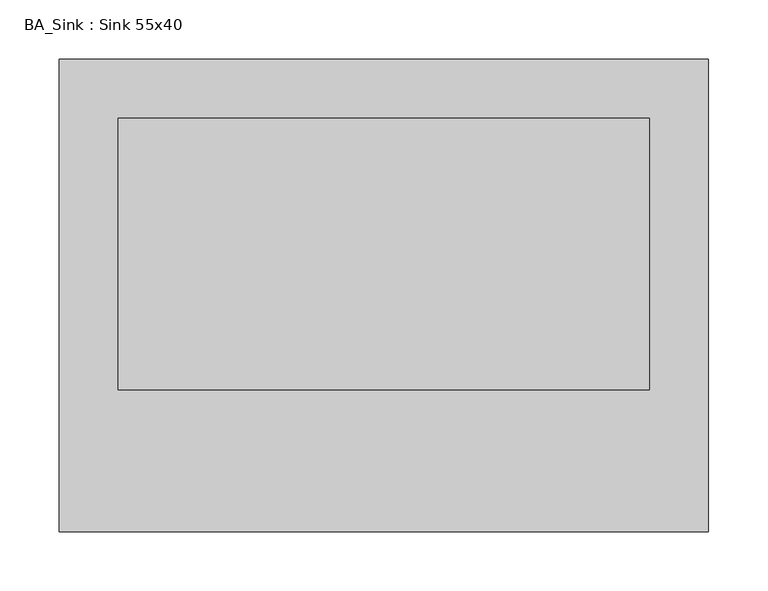
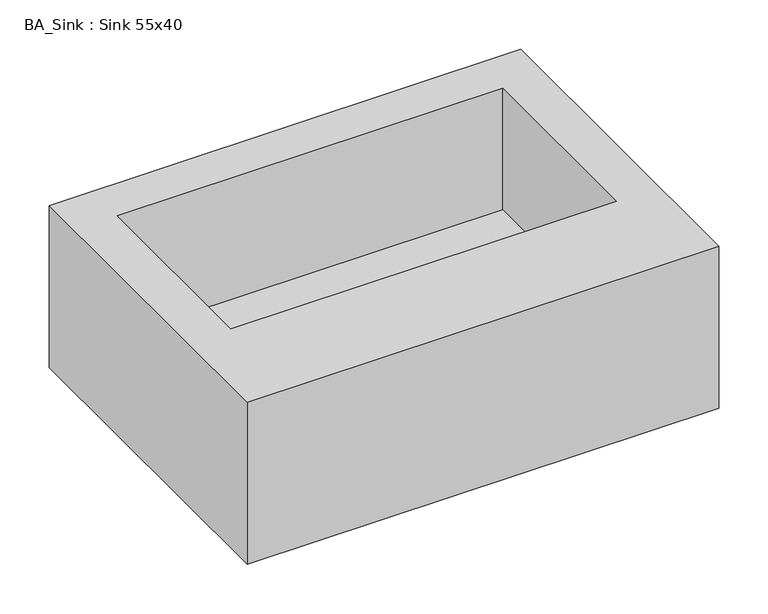
"""IFC4 building model written with IfcOpenShell, lengths in millimetres: flow terminal geometry, BA_Sink : Sink 55x40."""

from ifc_helpers import new_model, si_unit, origin, place, context, project, spatial, faceted_brep, source, transform, mapped, element, save


def ba_sink_sink_55x40_4eaba232(model_context):
    return source(origin(), model_context, "Body", "Brep", [
        faceted_brep([(400.0, 475.0, 900.0), (-150.0, 475.0, 900.0), (-150.0, 75.0, 900.0), (400.0, 75.0, 900.0), (-100.0, 425.0, 900.0), (350.0, 425.0, 900.0), (350.0, 195.0, 900.0), (-100.0, 195.0, 900.0), (400.0, 475.0, 700.0), (400.0, 75.0, 700.0), (-150.0, 75.0, 700.0), (-150.0, 475.0, 700.0), (350.0, 425.0, 750.0), (-100.0, 425.0, 750.0), (-100.0, 195.0, 750.0), (350.0, 195.0, 750.0)], [[[0, 1, 2, 3], [4, 5, 6, 7]], [[8, 9, 10, 11]], [[1, 0, 8, 11]], [[2, 1, 11, 10]], [[3, 2, 10, 9]], [[0, 3, 9, 8]], [[12, 13, 14, 15]], [[13, 12, 5, 4]], [[14, 13, 4, 7]], [[15, 14, 7, 6]], [[12, 15, 6, 5]]]),
    ])


if __name__ == "__main__":
    model = new_model("IFC4")
    model_context = context("Model", 3, world=origin())
    ifc_project = project(units=[si_unit("LENGTHUNIT", "METRE", prefix="MILLI")], contexts=[model_context])
    site = spatial("IfcSite", under=ifc_project)
    building = spatial("IfcBuilding", under=site)
    placement = place(None, origin())
    ba_sink_sink_55x40_shape = ba_sink_sink_55x40_4eaba232(model_context)
    element("IfcFlowTerminal", 1, ObjectType="BA_Sink : Sink 55x40", at=placement, inside=building, context=model_context, shape_type="MappedRepresentation", body=[
        mapped(ba_sink_sink_55x40_shape, transform((0.0, 0.0, 0.0), x_axis=(1.0, 0.0, 0.0), y_axis=(0.0, 1.0, 0.0), z_axis=(0.0, 0.0, 1.0))),
    ])
    save(model, "model.ifc")

# Revit data of these elements
# Type "BA_Sink : Sink 55x40"
#   height = 900 mm
#   width = 550 mm
#   depth = 400 mm
#   Default Elevation = 0
# Element 1 (IfcFlowTerminal, "BA_Sink : Sink 55x40")
#   Materials on its faces: "Default"
# Materials
#   "Default": class "Generic", colour RGB 255 255 255, transparency 0, Cost = 0
